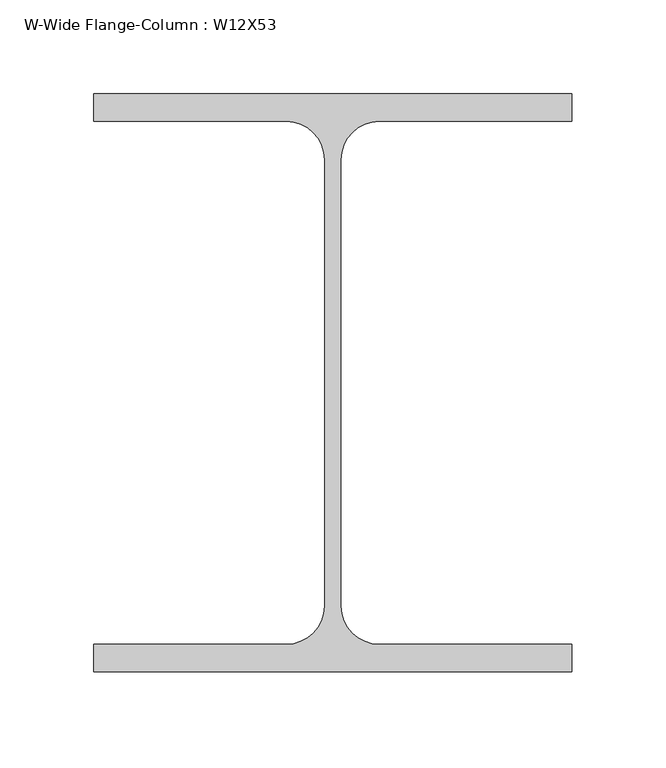
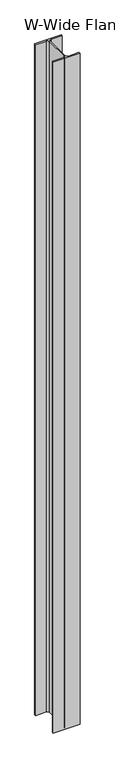
"""IFC4 building model written with IfcOpenShell, lengths in millimetres: column geometry, W-Wide Flange-Column : W12X53."""

import ifcopenshell
import ifcopenshell.guid

model = None  # the IFC model being written
_history = None  # IfcOwnerHistory: only IFC2X3 demands one
_inside = {}  # id of a spatial element -> (the spatial element, [elements in it])
_under = {}  # id of a project, library or spatial element -> (it, [spatial elements below it])
_declared = {}  # id of a project -> (the project, [libraries it declares])
_typed = {}  # id of a type object -> (the type object, [elements of that type])
_made_of = {}  # id of a material, layer set ... -> (it, [elements and type objects made of it])


def new_model(schema):
    """Start an empty IFC model of exactly this schema.

    Asked for "IFC4X3", IfcOpenShell would pick the latest addendum, in which some entities
    have other attributes; the version numbers below select the first issue.
    IFC2X3 requires an IfcOwnerHistory on every rooted entity: one is made here for all.
    """
    global model, _history
    if schema == "IFC4X3":
        model = ifcopenshell.file(schema_version=(4, 3, 0, 0))
    else:
        model = ifcopenshell.file(schema=schema)
    _inside.clear()
    _under.clear()
    _declared.clear()
    _typed.clear()
    _made_of.clear()
    _history = None
    if model.schema == "IFC2X3":
        org = make("IfcOrganization", Name="unknown")
        user = make(
            "IfcPersonAndOrganization",
            ThePerson=make("IfcPerson", FamilyName="unknown"),
            TheOrganization=org,
        )
        app = make(
            "IfcApplication",
            ApplicationDeveloper=org,
            Version="unknown",
            ApplicationFullName="unknown",
            ApplicationIdentifier="unknown",
        )
        _history = make(
            "IfcOwnerHistory",
            OwningUser=user,
            OwningApplication=app,
            ChangeAction="ADDED",
            CreationDate=0,
        )
    return model


def make(cls, **values):
    """One entity of the class cls with the attributes given. An attribute that is None is left unset."""
    return model.create_entity(
        cls, **{name: value for name, value in values.items() if value is not None}
    )


def rooted(cls, **values):
    """An entity with a GlobalId (a new one), such as an element, a storey or a relation."""
    return make(cls, GlobalId=ifcopenshell.guid.new(), OwnerHistory=_history, **values)


def si_unit(unit_type, name, prefix=None):
    """IfcSIUnit, for example si_unit("LENGTHUNIT", "METRE", prefix="MILLI")."""
    return make("IfcSIUnit", UnitType=unit_type, Prefix=prefix, Name=name)


def assignment(units):
    """IfcUnitAssignment: the units of a project."""
    return None if units is None else make("IfcUnitAssignment", Units=units)


def point(xyz):
    """IfcCartesianPoint."""
    return None if xyz is None else make("IfcCartesianPoint", Coordinates=xyz)


def direction(xyz):
    """IfcDirection."""
    return None if xyz is None else make("IfcDirection", DirectionRatios=xyz)


def frame(location, z_axis=None, x_axis=None):
    """IfcAxis2Placement3D, a coordinate frame: its origin and axes. An axis left out is left unset."""
    return make(
        "IfcAxis2Placement3D",
        Location=point(location),
        Axis=direction(z_axis),
        RefDirection=direction(x_axis),
    )


def frame_2d(location, x_axis=None):
    """IfcAxis2Placement2D, a coordinate frame in the plane: its origin and x axis."""
    return make(
        "IfcAxis2Placement2D", Location=point(location), RefDirection=direction(x_axis)
    )


def origin():
    """The frame at (0, 0, 0) with its axes left unset."""
    return frame((0.0, 0.0, 0.0))


def place(relative_to, where):
    """IfcLocalPlacement: puts the frame where relative to a parent placement (None: the world)."""
    return make(
        "IfcLocalPlacement", PlacementRelTo=relative_to, RelativePlacement=where
    )


def context(
    kind, dimensions, precision=None, world=None, true_north=None, identifier=None
):
    """IfcGeometricRepresentationContext, for example the 3D "Model" context."""
    return make(
        "IfcGeometricRepresentationContext",
        ContextIdentifier=identifier,
        ContextType=kind,
        CoordinateSpaceDimension=dimensions,
        Precision=precision,
        WorldCoordinateSystem=world,
        TrueNorth=true_north,
    )


def project(units=None, contexts=None):
    """IfcProject with its units and contexts."""
    return rooted(
        "IfcProject",
        Name="project",
        RepresentationContexts=contexts,
        UnitsInContext=assignment(units),
    )


def spatial(cls, under=None, at=None, **own):
    """A site, building, storey or space (cls), placed at a placement, below another one or the project."""
    s = rooted(cls, ObjectPlacement=at, **own)
    if under is not None:
        _under.setdefault(under.id(), (under, []))[1].append(s)
    return s


def polyline(points):
    """IfcPolyline through the points."""
    return make("IfcPolyline", Points=[point(p) for p in points])


def circle_curve(where, radius):
    """IfcCircle in the frame where."""
    return make("IfcCircle", Position=where, Radius=radius)


def trimmed(basis, trim1, trim2, sense, master):
    """IfcTrimmedCurve: the piece of a basis curve between two trims."""
    return make(
        "IfcTrimmedCurve",
        BasisCurve=basis,
        Trim1=trim1,
        Trim2=trim2,
        SenseAgreement=sense,
        MasterRepresentation=master,
    )


def segment(curve, same_sense, transition):
    """IfcCompositeCurveSegment."""
    return make(
        "IfcCompositeCurveSegment",
        Transition=transition,
        SameSense=same_sense,
        ParentCurve=curve,
    )


def composite_curve(segments, self_intersect=None):
    """IfcCompositeCurve: segments joined end to end."""
    return make("IfcCompositeCurve", Segments=segments, SelfIntersect=self_intersect)


def outline(outer, holes=None, kind="AREA"):
    """IfcArbitraryClosedProfileDef: a profile drawn as a closed curve; with holes, ...WithVoids."""
    if holes is None:
        return make("IfcArbitraryClosedProfileDef", ProfileType=kind, OuterCurve=outer)
    return make(
        "IfcArbitraryProfileDefWithVoids",
        ProfileType=kind,
        OuterCurve=outer,
        InnerCurves=holes,
    )


def extrude(swept, where, along, depth):
    """IfcExtrudedAreaSolid: the profile swept, set in the frame where, extruded along a direction by depth."""
    return make(
        "IfcExtrudedAreaSolid",
        SweptArea=swept,
        Position=where,
        ExtrudedDirection=direction(along),
        Depth=depth,
    )


def shape(context_of_items, identifier, shape_type, items):
    """IfcShapeRepresentation: the items that make up one representation, for example the "Body"."""
    return make(
        "IfcShapeRepresentation",
        ContextOfItems=context_of_items,
        RepresentationIdentifier=identifier,
        RepresentationType=shape_type,
        Items=items,
    )


def source(mapping_origin, context_of_items, identifier, shape_type, items):
    """IfcRepresentationMap: a shape defined once, which mapped items show again and again."""
    return make(
        "IfcRepresentationMap",
        MappingOrigin=mapping_origin,
        MappedRepresentation=shape(context_of_items, identifier, shape_type, items),
    )


def transform(
    local_origin,
    x_axis=None,
    y_axis=None,
    z_axis=None,
    scale=None,
    scale2=None,
    scale3=None,
    uniform=True,
):
    """IfcCartesianTransformationOperator3D, or its non-uniform kind. x_axis, y_axis, z_axis: its Axis1, 2, 3."""
    if uniform:
        return make(
            "IfcCartesianTransformationOperator3D",
            Axis1=direction(x_axis),
            Axis2=direction(y_axis),
            LocalOrigin=point(local_origin),
            Scale=scale,
            Axis3=direction(z_axis),
        )
    return make(
        "IfcCartesianTransformationOperator3DnonUniform",
        Axis1=direction(x_axis),
        Axis2=direction(y_axis),
        LocalOrigin=point(local_origin),
        Scale=scale,
        Axis3=direction(z_axis),
        Scale2=scale2,
        Scale3=scale3,
    )


def mapped(mapping_source, mapping_target):
    """IfcMappedItem: shows the shape of a source again, moved by a transform."""
    return make(
        "IfcMappedItem", MappingSource=mapping_source, MappingTarget=mapping_target
    )


def made_of(thing, what):
    """Note that an element or type object is made of a material, layer set ...; save() writes the relation."""
    if what is not None:
        _made_of.setdefault(what.id(), (what, []))[1].append(thing)
    return thing


def element(
    cls,
    number,
    at=None,
    inside=None,
    cuts=None,
    type_object=None,
    material=None,
    context=None,
    identifier="Body",
    shape_type=None,
    held_by="IfcProductDefinitionShape",
    body=None,
    shapes=None,
    **own,
):
    """One element of the class cls, such as IfcWall. Its Tag is "e" and its number.

    at: its placement. inside: the storey or other place that contains it. cuts: it is an
    opening in that element (IfcRelVoidsElement). A single representation is given by context,
    identifier, shape_type and body (its items); several are given by shapes. held_by: the class
    of the entity that holds the representations. save() writes the other relations.
    """
    e = rooted(cls, Tag="e%d" % number, ObjectPlacement=at, **own)
    if body is not None:
        shapes = [shape(context, identifier, shape_type, body)]
    if shapes is not None:
        e.Representation = make(held_by, Representations=shapes)
    if inside is not None:
        _inside.setdefault(inside.id(), (inside, []))[1].append(e)
    if cuts is not None:
        rooted(
            "IfcRelVoidsElement", RelatingBuildingElement=cuts, RelatedOpeningElement=e
        )
    if type_object is not None:
        _typed.setdefault(type_object.id(), (type_object, []))[1].append(e)
    return made_of(e, material)


def aggregate(whole, parts):
    """IfcRelAggregates: a whole, such as a stair, and the parts it consists of."""
    return rooted("IfcRelAggregates", RelatingObject=whole, RelatedObjects=parts)


def save(model, path):
    """Write the relations noted so far, then the file.

    IfcRelAggregates (storeys below a building ...), IfcRelContainedInSpatialStructure (elements
    in a storey), IfcRelDefinesByType, IfcRelAssociatesMaterial and IfcRelDeclares: one each for
    every whole, place, type object, material and project.
    """
    for whole, parts in _under.values():
        aggregate(whole, parts)
    for where, things in _inside.values():
        rooted(
            "IfcRelContainedInSpatialStructure",
            RelatedElements=things,
            RelatingStructure=where,
        )
    for kind, things in _typed.values():
        rooted("IfcRelDefinesByType", RelatedObjects=things, RelatingType=kind)
    for what, things in _made_of.values():
        rooted("IfcRelAssociatesMaterial", RelatedObjects=things, RelatingMaterial=what)
    for by, libraries in _declared.values():
        rooted("IfcRelDeclares", RelatingContext=by, RelatedDefinitions=libraries)
    model.write(path)


def w_wide_flange_column_w12x53_4b29bfd7(model_context):
    return source(origin(), model_context, "Body", "SweptSolid", [
        extrude(outline(composite_curve([segment(polyline([(127.0, 153.67), (127.0, 139.065), (24.7015, 139.065)]), True, "CONTINUOUS"), segment(trimmed(circle_curve(frame_2d((24.7015, 118.745)), 20.32), [point((24.7015, 139.065))], [point((4.3815, 118.745))], True, "CARTESIAN"), True, "CONTINUOUS"), segment(polyline([(4.3815, 118.745), (4.3815, -118.745)]), True, "CONTINUOUS"), segment(trimmed(circle_curve(frame_2d((24.7015, -118.745)), 20.32), [point((4.3815, -118.745))], [point((24.7015, -139.065))], True, "CARTESIAN"), True, "CONTINUOUS"), segment(polyline([(24.7015, -139.065), (127.0, -139.065), (127.0, -153.67), (-127.0, -153.67), (-127.0, -139.065), (-24.7015, -139.065)]), True, "CONTINUOUS"), segment(trimmed(circle_curve(frame_2d((-24.7015, -118.745)), 20.32), [point((-24.7015, -139.065))], [point((-4.3815, -118.745))], True, "CARTESIAN"), True, "CONTINUOUS"), segment(polyline([(-4.3815, -118.745), (-4.3815, 118.745)]), True, "CONTINUOUS"), segment(trimmed(circle_curve(frame_2d((-24.7015, 118.745)), 20.32), [point((-4.3815, 118.745))], [point((-24.7015, 139.065))], True, "CARTESIAN"), True, "CONTINUOUS"), segment(polyline([(-24.7015, 139.065), (-127.0, 139.065), (-127.0, 153.67), (127.0, 153.67)]), True, "CONTINUOUS")], self_intersect=False)), frame((0.0, 0.0, 8756.65), z_axis=(0.0, 0.0, 1.0), x_axis=(1.0, 0.0, 0.0)), (0.0, 0.0, 1.0), 6770.3898438),
    ])


if __name__ == "__main__":
    model = new_model("IFC4")
    model_context = context("Model", 3, world=origin())
    ifc_project = project(units=[si_unit("LENGTHUNIT", "METRE", prefix="MILLI")], contexts=[model_context])
    site = spatial("IfcSite", under=ifc_project)
    building = spatial("IfcBuilding", under=site)
    placement = place(None, origin())
    w_wide_flange_column_w12x53_shape = w_wide_flange_column_w12x53_4b29bfd7(model_context)
    element("IfcColumn", 1, ObjectType="W-Wide Flange-Column : W12X53", at=placement, inside=building, context=model_context, shape_type="MappedRepresentation", body=[
        mapped(w_wide_flange_column_w12x53_shape, transform((0.0, 0.0, 0.0), x_axis=(1.0, 0.0, 0.0), y_axis=(0.0, 1.0, 0.0), z_axis=(0.0, 0.0, 1.0))),
    ])
    save(model, "model.ifc")

# Revit data of these elements
# Type "W-Wide Flange-Column : W12X53"
#   Assembly Code = "B10"
#   W = 53
#   bf = 0' - 10"
#   d = 1' - 0.1"
#   k = 0' - 1 3/8"
#   kr = 0' - 0.8"
#   tf = 0' - 0.575"
#   tw = 0' - 0.345"
#   A = 0.108333 SF
#   Structural Material [instance default] = Steel ASTM A992
# Element 1 (IfcColumn, "W-Wide Flange-Column : W12X53")
#   Materials on its faces: "Steel ASTM A992"
# Materials
#   "Steel ASTM A992": class "Metal", colour RGB 199 199 199, transparency 0, Description = "Structural steel 50ksi", Cost = 0
